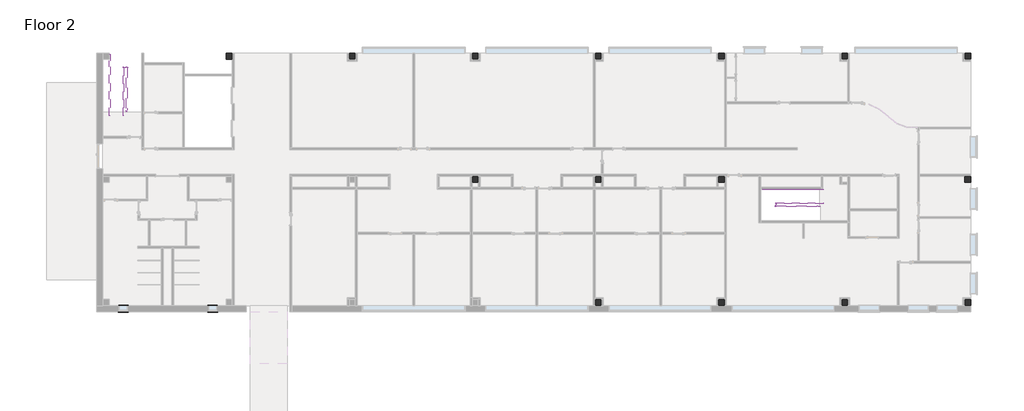
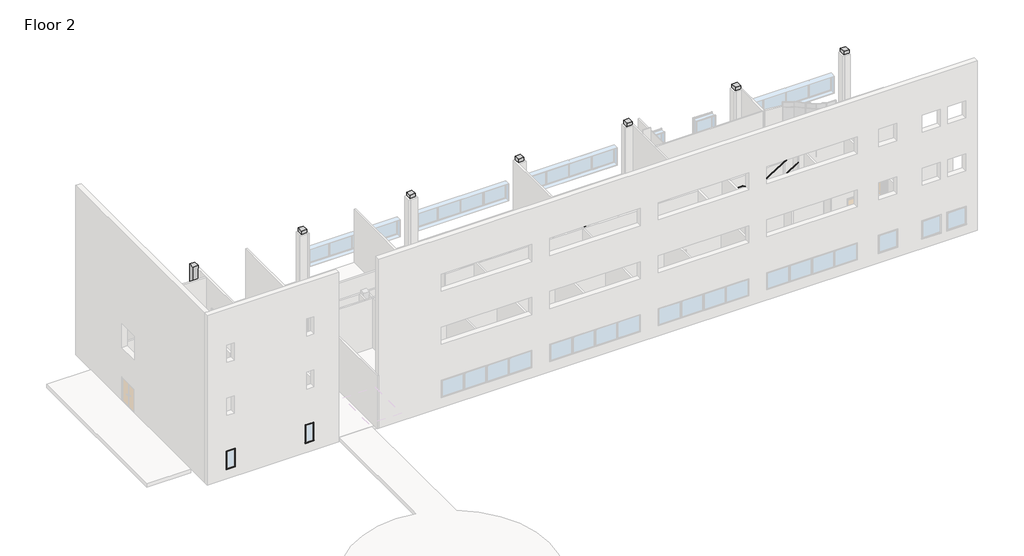
# One storey, part 5 of 7: 15 columns, 4 proxies, 4 railings.
"""IFC4 building model written with IfcOpenShell, lengths in millimetres."""

import ifcopenshell
import ifcopenshell.guid

model = None  # the IFC model being written
_history = None  # IfcOwnerHistory: only IFC2X3 demands one
_inside = {}  # id of a spatial element -> (the spatial element, [elements in it])
_under = {}  # id of a project, library or spatial element -> (it, [spatial elements below it])
_declared = {}  # id of a project -> (the project, [libraries it declares])
_typed = {}  # id of a type object -> (the type object, [elements of that type])
_made_of = {}  # id of a material, layer set ... -> (it, [elements and type objects made of it])


def new_model(schema):
    """Start an empty IFC model of exactly this schema.

    Asked for "IFC4X3", IfcOpenShell would pick the latest addendum, in which some entities
    have other attributes; the version numbers below select the first issue.
    IFC2X3 requires an IfcOwnerHistory on every rooted entity: one is made here for all.
    """
    global model, _history
    if schema == "IFC4X3":
        model = ifcopenshell.file(schema_version=(4, 3, 0, 0))
    else:
        model = ifcopenshell.file(schema=schema)
    _inside.clear()
    _under.clear()
    _declared.clear()
    _typed.clear()
    _made_of.clear()
    _history = None
    if model.schema == "IFC2X3":
        org = make("IfcOrganization", Name="unknown")
        user = make(
            "IfcPersonAndOrganization",
            ThePerson=make("IfcPerson", FamilyName="unknown"),
            TheOrganization=org,
        )
        app = make(
            "IfcApplication",
            ApplicationDeveloper=org,
            Version="unknown",
            ApplicationFullName="unknown",
            ApplicationIdentifier="unknown",
        )
        _history = make(
            "IfcOwnerHistory",
            OwningUser=user,
            OwningApplication=app,
            ChangeAction="ADDED",
            CreationDate=0,
        )
    return model


def make(cls, **values):
    """One entity of the class cls with the attributes given. An attribute that is None is left unset."""
    return model.create_entity(
        cls, **{name: value for name, value in values.items() if value is not None}
    )


def rooted(cls, **values):
    """An entity with a GlobalId (a new one), such as an element, a storey or a relation."""
    return make(cls, GlobalId=ifcopenshell.guid.new(), OwnerHistory=_history, **values)


def si_unit(unit_type, name, prefix=None):
    """IfcSIUnit, for example si_unit("LENGTHUNIT", "METRE", prefix="MILLI")."""
    return make("IfcSIUnit", UnitType=unit_type, Prefix=prefix, Name=name)


def assignment(units):
    """IfcUnitAssignment: the units of a project."""
    return None if units is None else make("IfcUnitAssignment", Units=units)


def point(xyz):
    """IfcCartesianPoint."""
    return None if xyz is None else make("IfcCartesianPoint", Coordinates=xyz)


def direction(xyz):
    """IfcDirection."""
    return None if xyz is None else make("IfcDirection", DirectionRatios=xyz)


def frame(location, z_axis=None, x_axis=None):
    """IfcAxis2Placement3D, a coordinate frame: its origin and axes. An axis left out is left unset."""
    return make(
        "IfcAxis2Placement3D",
        Location=point(location),
        Axis=direction(z_axis),
        RefDirection=direction(x_axis),
    )


def origin():
    """The frame at (0, 0, 0) with its axes left unset."""
    return frame((0.0, 0.0, 0.0))


def origin_with_axes():
    """The frame at (0, 0, 0) with the z axis (0, 0, 1) and the x axis (1, 0, 0) written out."""
    return frame((0.0, 0.0, 0.0), z_axis=(0.0, 0.0, 1.0), x_axis=(1.0, 0.0, 0.0))


def place(relative_to, where):
    """IfcLocalPlacement: puts the frame where relative to a parent placement (None: the world)."""
    return make(
        "IfcLocalPlacement", PlacementRelTo=relative_to, RelativePlacement=where
    )


def context(
    kind, dimensions, precision=None, world=None, true_north=None, identifier=None
):
    """IfcGeometricRepresentationContext, for example the 3D "Model" context."""
    return make(
        "IfcGeometricRepresentationContext",
        ContextIdentifier=identifier,
        ContextType=kind,
        CoordinateSpaceDimension=dimensions,
        Precision=precision,
        WorldCoordinateSystem=world,
        TrueNorth=true_north,
    )


def project(units=None, contexts=None):
    """IfcProject with its units and contexts."""
    return rooted(
        "IfcProject",
        Name="project",
        RepresentationContexts=contexts,
        UnitsInContext=assignment(units),
    )


def spatial(cls, under=None, at=None, **own):
    """A site, building, storey or space (cls), placed at a placement, below another one or the project."""
    s = rooted(cls, ObjectPlacement=at, **own)
    if under is not None:
        _under.setdefault(under.id(), (under, []))[1].append(s)
    return s


def polyline(points):
    """IfcPolyline through the points."""
    return make("IfcPolyline", Points=[point(p) for p in points])


def circle_curve(where, radius):
    """IfcCircle in the frame where."""
    return make("IfcCircle", Position=where, Radius=radius)


def outline(outer, holes=None, kind="AREA"):
    """IfcArbitraryClosedProfileDef: a profile drawn as a closed curve; with holes, ...WithVoids."""
    if holes is None:
        return make("IfcArbitraryClosedProfileDef", ProfileType=kind, OuterCurve=outer)
    return make(
        "IfcArbitraryProfileDefWithVoids",
        ProfileType=kind,
        OuterCurve=outer,
        InnerCurves=holes,
    )


def extrude(swept, where, along, depth):
    """IfcExtrudedAreaSolid: the profile swept, set in the frame where, extruded along a direction by depth."""
    return make(
        "IfcExtrudedAreaSolid",
        SweptArea=swept,
        Position=where,
        ExtrudedDirection=direction(along),
        Depth=depth,
    )


def faces_of(points, faces, orient=None, outer=None):
    """IfcFace entities. A face is a list of loops; a loop is a list of indices into points, from 0.

    orient and outer hold one flag for each loop. By default every Orientation is true, the
    first loop of a face is its IfcFaceOuterBound and the others are IfcFaceBound.
    """
    made = []
    for i, loops in enumerate(faces):
        bounds = []
        for j, loop in enumerate(loops):
            is_outer = j == 0 if outer is None else outer[i][j]
            bounds.append(
                make(
                    "IfcFaceOuterBound" if is_outer else "IfcFaceBound",
                    Bound=make("IfcPolyLoop", Polygon=[points[k] for k in loop]),
                    Orientation=True if orient is None else orient[i][j],
                )
            )
        made.append(make("IfcFace", Bounds=bounds))
    return made


def faceted_brep(points, faces, orient=None, outer=None, voids=None):
    """IfcFacetedBrep: a solid bounded by flat faces; with voids (closed shells), ...WithVoids."""
    shared = [point(p) for p in points]
    hull = make("IfcClosedShell", CfsFaces=faces_of(shared, faces, orient, outer))
    if voids is None:
        return make("IfcFacetedBrep", Outer=hull)
    return make(
        "IfcFacetedBrepWithVoids",
        Outer=hull,
        Voids=[
            make(cls, CfsFaces=faces_of(shared, fs, o, b)) for cls, fs, o, b in voids
        ],
    )


def shape(context_of_items, identifier, shape_type, items):
    """IfcShapeRepresentation: the items that make up one representation, for example the "Body"."""
    return make(
        "IfcShapeRepresentation",
        ContextOfItems=context_of_items,
        RepresentationIdentifier=identifier,
        RepresentationType=shape_type,
        Items=items,
    )


def source(mapping_origin, context_of_items, identifier, shape_type, items):
    """IfcRepresentationMap: a shape defined once, which mapped items show again and again."""
    return make(
        "IfcRepresentationMap",
        MappingOrigin=mapping_origin,
        MappedRepresentation=shape(context_of_items, identifier, shape_type, items),
    )


def transform(
    local_origin,
    x_axis=None,
    y_axis=None,
    z_axis=None,
    scale=None,
    scale2=None,
    scale3=None,
    uniform=True,
):
    """IfcCartesianTransformationOperator3D, or its non-uniform kind. x_axis, y_axis, z_axis: its Axis1, 2, 3."""
    if uniform:
        return make(
            "IfcCartesianTransformationOperator3D",
            Axis1=direction(x_axis),
            Axis2=direction(y_axis),
            LocalOrigin=point(local_origin),
            Scale=scale,
            Axis3=direction(z_axis),
        )
    return make(
        "IfcCartesianTransformationOperator3DnonUniform",
        Axis1=direction(x_axis),
        Axis2=direction(y_axis),
        LocalOrigin=point(local_origin),
        Scale=scale,
        Axis3=direction(z_axis),
        Scale2=scale2,
        Scale3=scale3,
    )


def mapped(mapping_source, mapping_target):
    """IfcMappedItem: shows the shape of a source again, moved by a transform."""
    return make(
        "IfcMappedItem", MappingSource=mapping_source, MappingTarget=mapping_target
    )


def made_of(thing, what):
    """Note that an element or type object is made of a material, layer set ...; save() writes the relation."""
    if what is not None:
        _made_of.setdefault(what.id(), (what, []))[1].append(thing)
    return thing


def element(
    cls,
    number,
    at=None,
    inside=None,
    cuts=None,
    type_object=None,
    material=None,
    context=None,
    identifier="Body",
    shape_type=None,
    held_by="IfcProductDefinitionShape",
    body=None,
    shapes=None,
    **own,
):
    """One element of the class cls, such as IfcWall. Its Tag is "e" and its number.

    at: its placement. inside: the storey or other place that contains it. cuts: it is an
    opening in that element (IfcRelVoidsElement). A single representation is given by context,
    identifier, shape_type and body (its items); several are given by shapes. held_by: the class
    of the entity that holds the representations. save() writes the other relations.
    """
    e = rooted(cls, Tag="e%d" % number, ObjectPlacement=at, **own)
    if body is not None:
        shapes = [shape(context, identifier, shape_type, body)]
    if shapes is not None:
        e.Representation = make(held_by, Representations=shapes)
    if inside is not None:
        _inside.setdefault(inside.id(), (inside, []))[1].append(e)
    if cuts is not None:
        rooted(
            "IfcRelVoidsElement", RelatingBuildingElement=cuts, RelatedOpeningElement=e
        )
    if type_object is not None:
        _typed.setdefault(type_object.id(), (type_object, []))[1].append(e)
    return made_of(e, material)


def aggregate(whole, parts):
    """IfcRelAggregates: a whole, such as a stair, and the parts it consists of."""
    return rooted("IfcRelAggregates", RelatingObject=whole, RelatedObjects=parts)


def save(model, path):
    """Write the relations noted so far, then the file.

    IfcRelAggregates (storeys below a building ...), IfcRelContainedInSpatialStructure (elements
    in a storey), IfcRelDefinesByType, IfcRelAssociatesMaterial and IfcRelDeclares: one each for
    every whole, place, type object, material and project.
    """
    for whole, parts in _under.values():
        aggregate(whole, parts)
    for where, things in _inside.values():
        rooted(
            "IfcRelContainedInSpatialStructure",
            RelatedElements=things,
            RelatingStructure=where,
        )
    for kind, things in _typed.values():
        rooted("IfcRelDefinesByType", RelatedObjects=things, RelatingType=kind)
    for what, things in _made_of.values():
        rooted("IfcRelAssociatesMaterial", RelatedObjects=things, RelatingMaterial=what)
    for by, libraries in _declared.values():
        rooted("IfcRelDeclares", RelatingContext=by, RelatedDefinitions=libraries)
    model.write(path)


def plane_surface(at):
    """IfcPlane: the flat surface through the origin of the frame at, square to its z axis."""
    return make("IfcPlane", Position=at)


def cylinder_surface(at, radius):
    """IfcCylindricalSurface: all points at the distance radius from the z axis of the frame at."""
    return make("IfcCylindricalSurface", Position=at, Radius=radius)


def advanced_brep(points, edges, surfaces, faces):
    """IfcAdvancedBrep: a solid bounded by faces that lie on surfaces and meet in shared edges.

    An edge is (start, end): straight between two places in points (the first is 0);
    or (start, end, curve); or (start, end, curve, False) where it runs against its curve.
    A face is (place in surfaces, loops), or (place, loops, False) where it looks against
    its surface's normal. A loop lists edges by number (the first is 1), with a minus sign
    where the edge is run from its end to its start. The first loop is the outer one.
    """
    corners = [point(p) for p in points]
    vertices = [make("IfcVertexPoint", VertexGeometry=c) for c in corners]
    made = []
    for start, end, *more in edges:
        made.append(
            make(
                "IfcEdgeCurve",
                EdgeStart=vertices[start],
                EdgeEnd=vertices[end],
                EdgeGeometry=more[0] if more else make("IfcPolyline", Points=[corners[start], corners[end]]),
                SameSense=more[1] if len(more) > 1 else True,
            )
        )
    hull = []
    for where, loops, *sense in faces:
        bounds = []
        for j, loop in enumerate(loops):
            ring = [make("IfcOrientedEdge", EdgeElement=made[abs(k) - 1], Orientation=k > 0) for k in loop]
            bounds.append(
                make(
                    "IfcFaceOuterBound" if j == 0 else "IfcFaceBound",
                    Bound=make("IfcEdgeLoop", EdgeList=ring),
                    Orientation=True,
                )
            )
        hull.append(make("IfcAdvancedFace", Bounds=bounds, FaceSurface=surfaces[where], SameSense=sense[0] if sense else True))
    return make("IfcAdvancedBrep", Outer=make("IfcClosedShell", CfsFaces=hull))


def trim_window_exterior_flat_with_sill_4912eb0d(model_context):
    return source(origin(), model_context, "Body", "SweptSolid", [
        extrude(outline(polyline([(361.95, -1546.1823709), (361.95, -1603.3323709), (-361.95, -1603.3323709), (-361.95, -1546.1823709), (361.95, -1546.1823709)])), origin_with_axes(), (0.0, 0.0, 1.0), 19.05),
        extrude(outline(polyline([(-1555.75, 38.1), (-1526.4580645, 38.1), (-1524.0, 19.05), (-1524.0, 0.0), (-1546.1823709, 0.0), (-1546.1823709, 19.05), (-1555.75, 19.05), (-1555.75, 38.1)])), frame((-374.65, 0.0, 0.0), z_axis=(1.0, 0.0, 0.0), x_axis=(0.0, 1.0, 0.0)), (0.0, 0.0, 1.0), 749.3),
        extrude(outline(polyline([(-361.95, 57.15), (361.95, 57.15), (361.95, -1524.0), (304.8, -1524.0), (304.8, 0.0), (-304.8, 0.0), (-304.8, -1524.0), (-361.95, -1524.0), (-361.95, 57.15)])), origin_with_axes(), (0.0, 0.0, 1.0), 19.05),
    ])


def trim_window_interior_flat_picture_frame_978fd00d(model_context):
    return source(origin(), model_context, "Body", "SweptSolid", [
        extrude(outline(polyline([(349.25, 44.45), (349.25, -1568.45), (-349.25, -1568.45), (-349.25, 44.45), (349.25, 44.45)]), holes=[polyline([(292.1, -12.7), (-292.1, -12.7), (-292.1, -1511.3), (292.1, -1511.3), (292.1, -12.7)])]), origin_with_axes(), (0.0, 0.0, 1.0), 31.75),
    ])


def stair_railing_1_d4a7e100(model_context):
    return source(origin(), model_context, "Body", "SolidModel", [
        faceted_brep([(-1415.3134126, 56357.2066802, 9028.2888889), (-1428.0134126, 56357.2066802, 9006.2918436), (-1453.4134126, 56357.2066802, 9006.2918436), (-1466.1134126, 56357.2066802, 9028.2888889), (-1453.4134126, 56357.2066802, 9050.2859341), (-1428.0134126, 56357.2066802, 9050.2859341), (-1415.3134126, 52725.0066802, 6753.5777778), (-1428.0134126, 52725.0066802, 6775.574823), (-1453.4134126, 52725.0066802, 6775.574823), (-1466.1134126, 52725.0066802, 6753.5777778), (-1453.4134126, 52725.0066802, 6731.5807325), (-1428.0134126, 52725.0066802, 6731.5807325)], [[[0, 1, 2, 3, 4, 5]], [[6, 7, 8, 9, 10, 11]], [[1, 0, 6, 11]], [[2, 1, 11, 10]], [[3, 2, 10, 9]], [[4, 3, 9, 8]], [[5, 4, 8, 7]], [[0, 5, 7, 6]]]),
        advanced_brep(
        [(-1136.9891104, 56281.0066802, 9028.2888889), (-1136.9891104, 56331.8066802, 9028.2888889), (-1491.5134126, 56281.0066802, 9028.2888889), (-1491.5134126, 56331.8066802, 9028.2888889)],
        [
            (0, 1, circle_curve(frame((-1136.9891104, 56306.4066802, 9028.2888889), z_axis=(1.0, 0.0, 0.0), x_axis=(0.0, -1.0, 0.0)), 25.4)),
            (1, 0, circle_curve(frame((-1136.9891104, 56306.4066802, 9028.2888889), z_axis=(1.0, 0.0, 0.0), x_axis=(0.0, -1.0, 0.0)), 25.4)),
            (2, 3, circle_curve(frame((-1491.5134126, 56306.4066802, 9028.2888889), z_axis=(-1.0, 0.0, 0.0), x_axis=(0.0, -1.0, 0.0)), 25.4)),
            (3, 2, circle_curve(frame((-1491.5134126, 56306.4066802, 9028.2888889), z_axis=(-1.0, 0.0, 0.0), x_axis=(0.0, -1.0, 0.0)), 25.4)),
            (0, 2),
            (3, 1),
        ],
        [
            plane_surface(frame((-1136.9891104, 56281.0066802, 9002.8888889), z_axis=(1.0, 0.0, 0.0), x_axis=(0.0, 1.0, 0.0))),
            plane_surface(frame((-1491.5134126, 56281.0066802, 9002.8888889), z_axis=(-1.0, 0.0, 0.0), x_axis=(0.0, -1.0, 0.0))),
            cylinder_surface(frame((-1491.5134126, 56306.4066802, 9028.2888889), z_axis=(1.0, 0.0, 0.0), x_axis=(0.0, -1.0, 0.0)), 25.4),
        ],
        [
            (0, [[1, 2]]),
            (1, [[3, 4]]),
            (2, [[-1, 5, -4, 6]]),
            (2, [[-2, -6, -3, -5]]),
        ],
    ),
        faceted_brep([(-1213.1891104, 53283.8066802, 11128.0222222), (-1200.4891104, 53283.8066802, 11106.025177), (-1175.0891104, 53283.8066802, 11106.025177), (-1162.3891104, 53283.8066802, 11128.0222222), (-1175.0891104, 53283.8066802, 11150.0192675), (-1200.4891104, 53283.8066802, 11150.0192675), (-1213.1891104, 56357.2066802, 9203.2666667), (-1200.4891104, 56357.2066802, 9225.2637119), (-1175.0891104, 56357.2066802, 9225.2637119), (-1162.3891104, 56357.2066802, 9203.2666667), (-1175.0891104, 56357.2066802, 9181.2696214), (-1200.4891104, 56357.2066802, 9181.2696214)], [[[0, 1, 2, 3, 4, 5]], [[6, 7, 8, 9, 10, 11]], [[1, 0, 6, 11]], [[2, 1, 11, 10]], [[3, 2, 10, 9]], [[4, 3, 9, 8]], [[5, 4, 8, 7]], [[0, 5, 7, 6]]]),
        faceted_brep([(-1213.1891104, 53004.4066802, 11303.0), (-1200.4891104, 53004.4066802, 11281.0029547), (-1175.0891104, 53004.4066802, 11281.0029547), (-1162.3891104, 53004.4066802, 11303.0), (-1175.0891104, 53004.4066802, 11324.9970453), (-1200.4891104, 53004.4066802, 11324.9970453), (-1213.1891104, 53283.8066802, 11128.0222222), (-1200.4891104, 53283.8066802, 11150.0192675), (-1175.0891104, 53283.8066802, 11150.0192675), (-1162.3891104, 53283.8066802, 11128.0222222), (-1175.0891104, 53283.8066802, 11106.025177), (-1200.4891104, 53283.8066802, 11106.025177)], [[[0, 1, 2, 3, 4, 5]], [[6, 7, 8, 9, 10, 11]], [[1, 0, 6, 11]], [[2, 1, 11, 10]], [[3, 2, 10, 9]], [[4, 3, 9, 8]], [[5, 4, 8, 7]], [[0, 5, 7, 6]]]),
    ])


def stair_railing_1_835fd4d1(model_context):
    return source(origin(), model_context, "Body", "SolidModel", [
        faceted_brep([(-2482.1134126, 56357.2066802, 9028.2888889), (-2469.4134126, 56357.2066802, 9050.2859341), (-2444.0134126, 56357.2066802, 9050.2859341), (-2431.3134126, 56357.2066802, 9028.2888889), (-2444.0134126, 56357.2066802, 9006.2918436), (-2469.4134126, 56357.2066802, 9006.2918436), (-2482.1134126, 52725.0066802, 6753.5777778), (-2469.4134126, 52725.0066802, 6731.5807325), (-2444.0134126, 52725.0066802, 6731.5807325), (-2431.3134126, 52725.0066802, 6753.5777778), (-2444.0134126, 52725.0066802, 6775.574823), (-2469.4134126, 52725.0066802, 6775.574823)], [[[0, 1, 2, 3, 4, 5]], [[6, 7, 8, 9, 10, 11]], [[1, 0, 6, 11]], [[2, 1, 11, 10]], [[3, 2, 10, 9]], [[4, 3, 9, 8]], [[5, 4, 8, 7]], [[0, 5, 7, 6]]]),
        advanced_brep(
        [(-2482.1134126, 57271.6066802, 9028.2888889), (-2431.3134126, 57271.6066802, 9028.2888889), (-2482.1134126, 56357.2066802, 9028.2888889), (-2431.3134126, 56357.2066802, 9028.2888889)],
        [
            (0, 1, circle_curve(frame((-2456.7134126, 57271.6066802, 9028.2888889), z_axis=(0.0, 1.0, 0.0), x_axis=(-0.9999999999999999, 0.0, 0.0)), 25.4)),
            (1, 0, circle_curve(frame((-2456.7134126, 57271.6066802, 9028.2888889), z_axis=(0.0, 1.0, 0.0), x_axis=(-0.9999999999999999, 0.0, 0.0)), 25.4)),
            (2, 3, circle_curve(frame((-2456.7134126, 56357.2066802, 9028.2888889), z_axis=(0.0, -1.0, 0.0), x_axis=(-0.9999999999999999, 0.0, 0.0)), 25.4)),
            (3, 2, circle_curve(frame((-2456.7134126, 56357.2066802, 9028.2888889), z_axis=(0.0, -1.0, 0.0), x_axis=(-0.9999999999999999, 0.0, 0.0)), 25.4)),
            (0, 2),
            (3, 1),
        ],
        [
            plane_surface(frame((-2482.1134126, 57271.6066802, 9002.8888889), z_axis=(0.0, 1.0, 0.0), x_axis=(0.0, 0.0, 1.0))),
            plane_surface(frame((-2482.1134126, 56357.2066802, 9002.8888889), z_axis=(0.0, -1.0, 0.0), x_axis=(0.0, 0.0, -1.0))),
            cylinder_surface(frame((-2456.7134126, 56357.2066802, 9028.2888889), z_axis=(0.0, 0.9999999999999999, 0.0), x_axis=(-0.9999999999999999, 0.0, 0.0)), 25.4),
        ],
        [
            (0, [[1, 2]]),
            (1, [[3, 4]]),
            (2, [[-1, 5, -4, 6]]),
            (2, [[-2, -6, -3, -5]]),
        ],
    ),
        advanced_brep(
        [(-222.5891104, 57347.8066802, 9028.2888889), (-222.5891104, 57297.0066802, 9028.2888889), (-2405.9134126, 57347.8066802, 9028.2888889), (-2405.9134126, 57297.0066802, 9028.2888889)],
        [
            (0, 1, circle_curve(frame((-222.5891104, 57322.4066802, 9028.2888889), z_axis=(1.0, 0.0, 0.0), x_axis=(0.0, 1.0, 0.0)), 25.4)),
            (1, 0, circle_curve(frame((-222.5891104, 57322.4066802, 9028.2888889), z_axis=(1.0, 0.0, 0.0), x_axis=(0.0, 1.0, 0.0)), 25.4)),
            (2, 3, circle_curve(frame((-2405.9134126, 57322.4066802, 9028.2888889), z_axis=(-1.0, 0.0, 0.0), x_axis=(0.0, 1.0, 0.0)), 25.4)),
            (3, 2, circle_curve(frame((-2405.9134126, 57322.4066802, 9028.2888889), z_axis=(-1.0, 0.0, 0.0), x_axis=(0.0, 1.0, 0.0)), 25.4)),
            (0, 2),
            (3, 1),
        ],
        [
            plane_surface(frame((-222.5891104, 57347.8066802, 9002.8888889), z_axis=(1.0, 0.0, 0.0), x_axis=(0.0, 1.0, 0.0))),
            plane_surface(frame((-2405.9134126, 57347.8066802, 9002.8888889), z_axis=(-1.0, 0.0, 0.0), x_axis=(0.0, -1.0, 0.0))),
            cylinder_surface(frame((-2405.9134126, 57322.4066802, 9028.2888889), z_axis=(1.0, 0.0, 0.0), x_axis=(0.0, 1.0, 0.0)), 25.4),
        ],
        [
            (0, [[1, 2]]),
            (1, [[3, 4]]),
            (2, [[-1, 5, -4, 6]]),
            (2, [[-2, -6, -3, -5]]),
        ],
    ),
        advanced_brep(
        [(-146.3891104, 56636.6066802, 9028.2888889), (-197.1891104, 56636.6066802, 9028.2888889), (-146.3891104, 57271.6066802, 9028.2888889), (-197.1891104, 57271.6066802, 9028.2888889)],
        [
            (0, 1, circle_curve(frame((-171.7891104, 56636.6066802, 9028.2888889), z_axis=(0.0, -1.0, 0.0), x_axis=(1.0, 0.0, 0.0)), 25.4)),
            (1, 0, circle_curve(frame((-171.7891104, 56636.6066802, 9028.2888889), z_axis=(0.0, -1.0, 0.0), x_axis=(1.0, 0.0, 0.0)), 25.4)),
            (2, 3, circle_curve(frame((-171.7891104, 57271.6066802, 9028.2888889), z_axis=(0.0, 1.0, 0.0), x_axis=(1.0, 0.0, 0.0)), 25.4)),
            (3, 2, circle_curve(frame((-171.7891104, 57271.6066802, 9028.2888889), z_axis=(0.0, 1.0, 0.0), x_axis=(1.0, 0.0, 0.0)), 25.4)),
            (0, 2),
            (3, 1),
        ],
        [
            plane_surface(frame((-146.3891104, 56636.6066802, 9002.8888889), z_axis=(0.0, -1.0, 0.0), x_axis=(0.0, 0.0, -1.0))),
            plane_surface(frame((-146.3891104, 57271.6066802, 9002.8888889), z_axis=(0.0, 1.0, 0.0), x_axis=(0.0, 0.0, 1.0))),
            cylinder_surface(frame((-171.7891104, 57271.6066802, 9028.2888889), z_axis=(0.0, -1.0, 0.0), x_axis=(1.0, 0.0, 0.0)), 25.4),
        ],
        [
            (0, [[1, 2]]),
            (1, [[3, 4]]),
            (2, [[-1, 5, -4, 6]]),
            (2, [[-2, -6, -3, -5]]),
        ],
    ),
        faceted_brep([(-146.3891104, 56357.2066802, 9203.2666667), (-159.0891104, 56357.2066802, 9225.2637119), (-184.4891104, 56357.2066802, 9225.2637119), (-197.1891104, 56357.2066802, 9203.2666667), (-184.4891104, 56357.2066802, 9181.2696214), (-159.0891104, 56357.2066802, 9181.2696214), (-146.3891104, 56636.6066802, 9028.2888889), (-159.0891104, 56636.6066802, 9006.2918436), (-184.4891104, 56636.6066802, 9006.2918436), (-197.1891104, 56636.6066802, 9028.2888889), (-184.4891104, 56636.6066802, 9050.2859341), (-159.0891104, 56636.6066802, 9050.2859341)], [[[0, 1, 2, 3, 4, 5]], [[6, 7, 8, 9, 10, 11]], [[1, 0, 6, 11]], [[2, 1, 11, 10]], [[3, 2, 10, 9]], [[4, 3, 9, 8]], [[5, 4, 8, 7]], [[0, 5, 7, 6]]]),
        faceted_brep([(-146.3891104, 53283.8066802, 11128.0222222), (-159.0891104, 53283.8066802, 11150.0192675), (-184.4891104, 53283.8066802, 11150.0192675), (-197.1891104, 53283.8066802, 11128.0222222), (-184.4891104, 53283.8066802, 11106.025177), (-159.0891104, 53283.8066802, 11106.025177), (-146.3891104, 56357.2066802, 9203.2666667), (-159.0891104, 56357.2066802, 9181.2696214), (-184.4891104, 56357.2066802, 9181.2696214), (-197.1891104, 56357.2066802, 9203.2666667), (-184.4891104, 56357.2066802, 9225.2637119), (-159.0891104, 56357.2066802, 9225.2637119)], [[[0, 1, 2, 3, 4, 5]], [[6, 7, 8, 9, 10, 11]], [[1, 0, 6, 11]], [[2, 1, 11, 10]], [[3, 2, 10, 9]], [[4, 3, 9, 8]], [[5, 4, 8, 7]], [[0, 5, 7, 6]]]),
        faceted_brep([(-146.3891104, 53004.4066802, 11303.0), (-159.0891104, 53004.4066802, 11324.9970453), (-184.4891104, 53004.4066802, 11324.9970453), (-197.1891104, 53004.4066802, 11303.0), (-184.4891104, 53004.4066802, 11281.0029547), (-159.0891104, 53004.4066802, 11281.0029547), (-146.3891104, 53283.8066802, 11128.0222222), (-159.0891104, 53283.8066802, 11106.025177), (-184.4891104, 53283.8066802, 11106.025177), (-197.1891104, 53283.8066802, 11128.0222222), (-184.4891104, 53283.8066802, 11150.0192675), (-159.0891104, 53283.8066802, 11150.0192675)], [[[0, 1, 2, 3, 4, 5]], [[6, 7, 8, 9, 10, 11]], [[1, 0, 6, 11]], [[2, 1, 11, 10]], [[3, 2, 10, 9]], [[4, 3, 9, 8]], [[5, 4, 8, 7]], [[0, 5, 7, 6]]]),
    ])


def stair_railing_1_a30edcdb(model_context):
    return source(origin(), model_context, "Body", "SolidModel", [
        faceted_brep([(46974.7398084, 47258.2865351, 9028.2888889), (46974.7398084, 47245.5865351, 9006.2918436), (46974.7398084, 47220.1865351, 9006.2918436), (46974.7398084, 47207.4865351, 9028.2888889), (46974.7398084, 47220.1865351, 9050.2859341), (46974.7398084, 47245.5865351, 9050.2859341), (50533.2139908, 47258.2865351, 6753.5777778), (50533.2139908, 47245.5865351, 6775.574823), (50533.2139908, 47220.1865351, 6775.574823), (50533.2139908, 47207.4865351, 6753.5777778), (50533.2139908, 47220.1865351, 6731.5807325), (50533.2139908, 47245.5865351, 6731.5807325)], [[[0, 1, 2, 3, 4, 5]], [[6, 7, 8, 9, 10, 11]], [[1, 0, 6, 11]], [[2, 1, 11, 10]], [[3, 2, 10, 9]], [[4, 3, 9, 8]], [[5, 4, 8, 7]], [[0, 5, 7, 6]]]),
        advanced_brep(
        [(46060.3398084, 47258.2865351, 9028.2888889), (46060.3398084, 47207.4865351, 9028.2888889), (46974.7398084, 47258.2865351, 9028.2888889), (46974.7398084, 47207.4865351, 9028.2888889)],
        [
            (0, 1, circle_curve(frame((46060.3398084, 47232.8865351, 9028.2888889), z_axis=(-1.0, 0.0, 0.0), x_axis=(0.0, 1.0, 0.0)), 25.4)),
            (1, 0, circle_curve(frame((46060.3398084, 47232.8865351, 9028.2888889), z_axis=(-1.0, 0.0, 0.0), x_axis=(0.0, 1.0, 0.0)), 25.4)),
            (2, 3, circle_curve(frame((46974.7398084, 47232.8865351, 9028.2888889), z_axis=(1.0, 0.0, 0.0), x_axis=(0.0, 1.0, 0.0)), 25.4)),
            (3, 2, circle_curve(frame((46974.7398084, 47232.8865351, 9028.2888889), z_axis=(1.0, 0.0, 0.0), x_axis=(0.0, 1.0, 0.0)), 25.4)),
            (0, 2),
            (3, 1),
        ],
        [
            plane_surface(frame((46060.3398084, 47258.2865351, 9002.8888889), z_axis=(-1.0, 0.0, 0.0), x_axis=(0.0, -1.0, 0.0))),
            plane_surface(frame((46974.7398084, 47258.2865351, 9002.8888889), z_axis=(1.0, 0.0, 0.0), x_axis=(0.0, 1.0, 0.0))),
            cylinder_surface(frame((46974.7398084, 47232.8865351, 9028.2888889), z_axis=(-1.0, 0.0, 0.0), x_axis=(0.0, 1.0, 0.0)), 25.4),
        ],
        [
            (0, [[1, 2]]),
            (1, [[3, 4]]),
            (2, [[-1, 5, -4, 6]]),
            (2, [[-2, -6, -3, -5]]),
        ],
    ),
        advanced_brep(
        [(45984.1398084, 45032.0030566, 9028.2888889), (46034.9398084, 45032.0030566, 9028.2888889), (45984.1398084, 47182.0865351, 9028.2888889), (46034.9398084, 47182.0865351, 9028.2888889)],
        [
            (0, 1, circle_curve(frame((46009.5398084, 45032.0030566, 9028.2888889), z_axis=(0.0, -1.0, 0.0), x_axis=(-1.0, 0.0, 0.0)), 25.4)),
            (1, 0, circle_curve(frame((46009.5398084, 45032.0030566, 9028.2888889), z_axis=(0.0, -1.0, 0.0), x_axis=(-1.0, 0.0, 0.0)), 25.4)),
            (2, 3, circle_curve(frame((46009.5398084, 47182.0865351, 9028.2888889), z_axis=(0.0, 1.0, 0.0), x_axis=(-1.0, 0.0, 0.0)), 25.4)),
            (3, 2, circle_curve(frame((46009.5398084, 47182.0865351, 9028.2888889), z_axis=(0.0, 1.0, 0.0), x_axis=(-1.0, 0.0, 0.0)), 25.4)),
            (0, 2),
            (3, 1),
        ],
        [
            plane_surface(frame((45984.1398084, 45032.0030566, 9002.8888889), z_axis=(0.0, -1.0, 0.0), x_axis=(0.0, 0.0, -1.0))),
            plane_surface(frame((45984.1398084, 47182.0865351, 9002.8888889), z_axis=(0.0, 1.0, 0.0), x_axis=(0.0, 0.0, 1.0))),
            cylinder_surface(frame((46009.5398084, 47182.0865351, 9028.2888889), z_axis=(0.0, -1.0, 0.0), x_axis=(-1.0, 0.0, 0.0)), 25.4),
        ],
        [
            (0, [[1, 2]]),
            (1, [[3, 4]]),
            (2, [[-1, 5, -4, 6]]),
            (2, [[-2, -6, -3, -5]]),
        ],
    ),
        advanced_brep(
        [(46695.3398084, 44955.8030566, 9028.2888889), (46695.3398084, 45006.6030566, 9028.2888889), (46060.3398084, 44955.8030566, 9028.2888889), (46060.3398084, 45006.6030566, 9028.2888889)],
        [
            (0, 1, circle_curve(frame((46695.3398084, 44981.2030566, 9028.2888889), z_axis=(1.0, 0.0, 0.0), x_axis=(0.0, -1.0, 0.0)), 25.4)),
            (1, 0, circle_curve(frame((46695.3398084, 44981.2030566, 9028.2888889), z_axis=(1.0, 0.0, 0.0), x_axis=(0.0, -1.0, 0.0)), 25.4)),
            (2, 3, circle_curve(frame((46060.3398084, 44981.2030566, 9028.2888889), z_axis=(-1.0, 0.0, 0.0), x_axis=(0.0, -1.0, 0.0)), 25.4)),
            (3, 2, circle_curve(frame((46060.3398084, 44981.2030566, 9028.2888889), z_axis=(-1.0, 0.0, 0.0), x_axis=(0.0, -1.0, 0.0)), 25.4)),
            (0, 2),
            (3, 1),
        ],
        [
            plane_surface(frame((46695.3398084, 44955.8030566, 9002.8888889), z_axis=(1.0, 0.0, 0.0), x_axis=(0.0, 1.0, 0.0))),
            plane_surface(frame((46060.3398084, 44955.8030566, 9002.8888889), z_axis=(-1.0, 0.0, 0.0), x_axis=(0.0, -1.0, 0.0))),
            cylinder_surface(frame((46060.3398084, 44981.2030566, 9028.2888889), z_axis=(1.0, 0.0, 0.0), x_axis=(0.0, -1.0, 0.0)), 25.4),
        ],
        [
            (0, [[1, 2]]),
            (1, [[3, 4]]),
            (2, [[-1, 5, -4, 6]]),
            (2, [[-2, -6, -3, -5]]),
        ],
    ),
        faceted_brep([(46974.7398084, 44955.8030566, 9203.2666667), (46974.7398084, 44968.5030566, 9181.2696214), (46974.7398084, 44993.9030566, 9181.2696214), (46974.7398084, 45006.6030566, 9203.2666667), (46974.7398084, 44993.9030566, 9225.2637119), (46974.7398084, 44968.5030566, 9225.2637119), (46695.3398084, 44955.8030566, 9028.2888889), (46695.3398084, 44968.5030566, 9050.2859341), (46695.3398084, 44993.9030566, 9050.2859341), (46695.3398084, 45006.6030566, 9028.2888889), (46695.3398084, 44993.9030566, 9006.2918436), (46695.3398084, 44968.5030566, 9006.2918436)], [[[0, 1, 2, 3, 4, 5]], [[6, 7, 8, 9, 10, 11]], [[1, 0, 6, 11]], [[2, 1, 11, 10]], [[3, 2, 10, 9]], [[4, 3, 9, 8]], [[5, 4, 8, 7]], [[0, 5, 7, 6]]]),
        faceted_brep([(50048.1398084, 44955.8030566, 11128.0222222), (50048.1398084, 44968.5030566, 11106.025177), (50048.1398084, 44993.9030566, 11106.025177), (50048.1398084, 45006.6030566, 11128.0222222), (50048.1398084, 44993.9030566, 11150.0192675), (50048.1398084, 44968.5030566, 11150.0192675), (46974.7398084, 44955.8030566, 9203.2666667), (46974.7398084, 44968.5030566, 9225.2637119), (46974.7398084, 44993.9030566, 9225.2637119), (46974.7398084, 45006.6030566, 9203.2666667), (46974.7398084, 44993.9030566, 9181.2696214), (46974.7398084, 44968.5030566, 9181.2696214)], [[[0, 1, 2, 3, 4, 5]], [[6, 7, 8, 9, 10, 11]], [[1, 0, 6, 11]], [[2, 1, 11, 10]], [[3, 2, 10, 9]], [[4, 3, 9, 8]], [[5, 4, 8, 7]], [[0, 5, 7, 6]]]),
        faceted_brep([(50327.5398084, 44955.8030566, 11303.0), (50327.5398084, 44968.5030566, 11281.0029547), (50327.5398084, 44993.9030566, 11281.0029547), (50327.5398084, 45006.6030566, 11303.0), (50327.5398084, 44993.9030566, 11324.9970453), (50327.5398084, 44968.5030566, 11324.9970453), (50048.1398084, 44955.8030566, 11128.0222222), (50048.1398084, 44968.5030566, 11150.0192675), (50048.1398084, 44993.9030566, 11150.0192675), (50048.1398084, 45006.6030566, 11128.0222222), (50048.1398084, 44993.9030566, 11106.025177), (50048.1398084, 44968.5030566, 11106.025177)], [[[0, 1, 2, 3, 4, 5]], [[6, 7, 8, 9, 10, 11]], [[1, 0, 6, 11]], [[2, 1, 11, 10]], [[3, 2, 10, 9]], [[4, 3, 9, 8]], [[5, 4, 8, 7]], [[0, 5, 7, 6]]]),
    ])


def stair_railing_1_ea28da98(model_context):
    return source(origin(), model_context, "Body", "SolidModel", [
        faceted_brep([(46974.7398084, 46191.4865351, 9028.2888889), (46974.7398084, 46204.1865351, 9050.2859341), (46974.7398084, 46229.5865351, 9050.2859341), (46974.7398084, 46242.2865351, 9028.2888889), (46974.7398084, 46229.5865351, 9006.2918436), (46974.7398084, 46204.1865351, 9006.2918436), (50533.2139908, 46191.4865351, 6753.5777778), (50533.2139908, 46204.1865351, 6731.5807325), (50533.2139908, 46229.5865351, 6731.5807325), (50533.2139908, 46242.2865351, 6753.5777778), (50533.2139908, 46229.5865351, 6775.574823), (50533.2139908, 46204.1865351, 6775.574823)], [[[0, 1, 2, 3, 4, 5]], [[6, 7, 8, 9, 10, 11]], [[1, 0, 6, 11]], [[2, 1, 11, 10]], [[3, 2, 10, 9]], [[4, 3, 9, 8]], [[5, 4, 8, 7]], [[0, 5, 7, 6]]]),
        advanced_brep(
        [(47050.9398084, 45946.4030566, 9028.2888889), (47000.1398084, 45946.4030566, 9028.2888889), (47050.9398084, 46267.6865351, 9028.2888889), (47000.1398084, 46267.6865351, 9028.2888889)],
        [
            (0, 1, circle_curve(frame((47025.5398084, 45946.4030566, 9028.2888889), z_axis=(0.0, -1.0, 0.0), x_axis=(1.0, 0.0, 0.0)), 25.4)),
            (1, 0, circle_curve(frame((47025.5398084, 45946.4030566, 9028.2888889), z_axis=(0.0, -1.0, 0.0), x_axis=(1.0, 0.0, 0.0)), 25.4)),
            (2, 3, circle_curve(frame((47025.5398084, 46267.6865351, 9028.2888889), z_axis=(0.0, 1.0, 0.0), x_axis=(1.0, 0.0, 0.0)), 25.4)),
            (3, 2, circle_curve(frame((47025.5398084, 46267.6865351, 9028.2888889), z_axis=(0.0, 1.0, 0.0), x_axis=(1.0, 0.0, 0.0)), 25.4)),
            (0, 2),
            (3, 1),
        ],
        [
            plane_surface(frame((47050.9398084, 45946.4030566, 9002.8888889), z_axis=(0.0, -1.0, 0.0), x_axis=(0.0, 0.0, -1.0))),
            plane_surface(frame((47050.9398084, 46267.6865351, 9002.8888889), z_axis=(0.0, 1.0, 0.0), x_axis=(0.0, 0.0, 1.0))),
            cylinder_surface(frame((47025.5398084, 46267.6865351, 9028.2888889), z_axis=(0.0, -1.0, 0.0), x_axis=(1.0, 0.0, 0.0)), 25.4),
        ],
        [
            (0, [[1, 2]]),
            (1, [[3, 4]]),
            (2, [[-1, 5, -4, 6]]),
            (2, [[-2, -6, -3, -5]]),
        ],
    ),
        faceted_brep([(50048.1398084, 46022.6030566, 11128.0222222), (50048.1398084, 46009.9030566, 11150.0192675), (50048.1398084, 45984.5030566, 11150.0192675), (50048.1398084, 45971.8030566, 11128.0222222), (50048.1398084, 45984.5030566, 11106.025177), (50048.1398084, 46009.9030566, 11106.025177), (46974.7398084, 46022.6030566, 9203.2666667), (46974.7398084, 46009.9030566, 9181.2696214), (46974.7398084, 45984.5030566, 9181.2696214), (46974.7398084, 45971.8030566, 9203.2666667), (46974.7398084, 45984.5030566, 9225.2637119), (46974.7398084, 46009.9030566, 9225.2637119)], [[[0, 1, 2, 3, 4, 5]], [[6, 7, 8, 9, 10, 11]], [[1, 0, 6, 11]], [[2, 1, 11, 10]], [[3, 2, 10, 9]], [[4, 3, 9, 8]], [[5, 4, 8, 7]], [[0, 5, 7, 6]]]),
        faceted_brep([(50327.5398084, 46022.6030566, 11303.0), (50327.5398084, 46009.9030566, 11324.9970453), (50327.5398084, 45984.5030566, 11324.9970453), (50327.5398084, 45971.8030566, 11303.0), (50327.5398084, 45984.5030566, 11281.0029547), (50327.5398084, 46009.9030566, 11281.0029547), (50048.1398084, 46022.6030566, 11128.0222222), (50048.1398084, 46009.9030566, 11106.025177), (50048.1398084, 45984.5030566, 11106.025177), (50048.1398084, 45971.8030566, 11128.0222222), (50048.1398084, 45984.5030566, 11150.0192675), (50048.1398084, 46009.9030566, 11150.0192675)], [[[0, 1, 2, 3, 4, 5]], [[6, 7, 8, 9, 10, 11]], [[1, 0, 6, 11]], [[2, 1, 11, 10]], [[3, 2, 10, 9]], [[4, 3, 9, 8]], [[5, 4, 8, 7]], [[0, 5, 7, 6]]]),
    ])


model = new_model("IFC4")

# Units and contexts
model_context = context("Model", 3, world=origin())
ifc_project = project(units=[si_unit("LENGTHUNIT", "METRE", prefix="MILLI")], contexts=[model_context])

# Site, building, storey
site = spatial("IfcSite", under=ifc_project)
building = spatial("IfcBuilding", under=site)
storey = spatial("IfcBuildingStorey", under=building, Name="Floor 2", Elevation=5486.4)

# Proxies
placement = place(None, origin())
trim_window_exterior_flat_with_sill_shape = trim_window_exterior_flat_with_sill_4912eb0d(model_context)
element("IfcBuildingElementProxy", 1, Name="Trim-Window-Exterior-Flat : with Sill", ObjectType="Trim-Window-Exterior-Flat : with Sill", at=placement, inside=storey, context=model_context, shape_type="MappedRepresentation", body=[
    mapped(trim_window_exterior_flat_with_sill_shape, transform((-1446.1807976, 38164.299389, 7924.8), x_axis=(1.0, 0.0, 0.0), y_axis=(0.0, 0.0, 1.0), z_axis=(0.0, -1.0, 0.0))),
])
element("IfcBuildingElementProxy", 2, Name="Trim-Window-Exterior-Flat : with Sill", ObjectType="Trim-Window-Exterior-Flat : with Sill", at=placement, inside=storey, context=model_context, shape_type="MappedRepresentation", body=[
    mapped(trim_window_exterior_flat_with_sill_shape, transform((5189.5692024, 38164.299389, 7924.8), x_axis=(1.0, 0.0, 0.0), y_axis=(0.0, 0.0, 1.0), z_axis=(0.0, -1.0, 0.0))),
])
trim_window_interior_flat_picture_frame_shape = trim_window_interior_flat_picture_frame_978fd00d(model_context)
element("IfcBuildingElementProxy", 3, Name="Trim-Window-Interior-Flat : Picture Frame", ObjectType="Trim-Window-Interior-Flat : Picture Frame", at=placement, inside=storey, context=model_context, shape_type="MappedRepresentation", body=[
    mapped(trim_window_interior_flat_picture_frame_shape, transform((-1446.1807976, 38618.324389, 7924.8), x_axis=(-1.0, 0.0, 0.0), y_axis=(0.0, 0.0, 1.0), z_axis=(0.0, 1.0, 0.0))),
])
element("IfcBuildingElementProxy", 4, Name="Trim-Window-Interior-Flat : Picture Frame", ObjectType="Trim-Window-Interior-Flat : Picture Frame", at=placement, inside=storey, context=model_context, shape_type="MappedRepresentation", body=[
    mapped(trim_window_interior_flat_picture_frame_shape, transform((5189.5692024, 38618.324389, 7924.8), x_axis=(-1.0, 0.0, 0.0), y_axis=(0.0, 0.0, 1.0), z_axis=(0.0, 1.0, 0.0))),
])

# Columns
element("IfcColumn", 5, ObjectType="Rectangular Column1 : 18\" x 18\"", at=placement, inside=storey, context=model_context, shape_type="Brep", body=[
    faceted_brep([(34069.3692024, 39077.111889, 10210.8), (33612.1692024, 39077.111889, 10210.8), (33612.1692024, 38619.911889, 10210.8), (34069.3692024, 38619.911889, 10210.8), (34069.3692024, 39077.111889, 5486.4), (34069.3692024, 38619.911889, 5486.4), (33612.1692024, 38619.911889, 5486.4), (33612.1692024, 39077.111889, 5486.4), (34069.3692024, 39077.111889, 9906.0), (33612.1692024, 39077.111889, 9906.0)], [[[0, 1, 2, 3]], [[4, 5, 6, 7]], [[1, 0, 8, 4, 7, 9]], [[2, 1, 9, 7, 6]], [[3, 2, 6, 5]], [[0, 3, 5, 4, 8]]]),
])
element("IfcColumn", 6, ObjectType="Rectangular Column1 : 18\" x 18\"", at=placement, inside=storey, context=model_context, shape_type="Brep", body=[
    faceted_brep([(43213.3692024, 39077.111889, 10210.8), (42756.1692024, 39077.111889, 10210.8), (42756.1692024, 38619.911889, 10210.8), (43213.3692024, 38619.911889, 10210.8), (43213.3692024, 39077.111889, 5486.4), (43213.3692024, 38619.911889, 5486.4), (42756.1692024, 38619.911889, 5486.4), (42756.1692024, 39077.111889, 5486.4), (43213.3692024, 39077.111889, 9906.0), (42756.1692024, 39077.111889, 9906.0)], [[[0, 1, 2, 3]], [[4, 5, 6, 7]], [[1, 0, 8, 4, 7, 9]], [[2, 1, 9, 7, 6]], [[3, 2, 6, 5]], [[0, 3, 5, 4, 8]]]),
])
element("IfcColumn", 7, ObjectType="Rectangular Column1 : 18\" x 18\"", at=placement, inside=storey, context=model_context, shape_type="Brep", body=[
    faceted_brep([(52357.3692024, 39077.111889, 10210.8), (51900.1692024, 39077.111889, 10210.8), (51900.1692024, 38619.911889, 10210.8), (52357.3692024, 38619.911889, 10210.8), (52357.3692024, 39077.111889, 5486.4), (52357.3692024, 38619.911889, 5486.4), (51900.1692024, 38619.911889, 5486.4), (51900.1692024, 39077.111889, 5486.4), (52357.3692024, 39077.111889, 9906.0), (51900.1692024, 39077.111889, 9906.0)], [[[0, 1, 2, 3]], [[4, 5, 6, 7]], [[1, 0, 8, 4, 7, 9]], [[2, 1, 9, 7, 6]], [[3, 2, 6, 5]], [[0, 3, 5, 4, 8]]]),
])
element("IfcColumn", 8, ObjectType="Rectangular Column1 : 18\" x 18\"", at=placement, inside=storey, context=model_context, shape_type="Brep", body=[
    faceted_brep([(61501.3692024, 39077.111889, 10210.8), (61044.1692024, 39077.111889, 10210.8), (61044.1692024, 38619.911889, 10210.8), (61501.3692024, 38619.911889, 10210.8), (61501.3692024, 39077.111889, 5486.4), (61501.3692024, 38619.911889, 5486.4), (61044.1692024, 38619.911889, 5486.4), (61044.1692024, 39077.111889, 5486.4), (61044.1692024, 39077.111889, 9906.0)], [[[0, 1, 2, 3]], [[4, 5, 6, 7]], [[1, 0, 4, 7, 8]], [[2, 1, 8, 7, 6]], [[3, 2, 6, 5]], [[0, 3, 5, 4]]]),
])
element("IfcColumn", 9, ObjectType="Rectangular Column1 : 18\" x 18\"", at=placement, inside=storey, context=model_context, shape_type="Brep", body=[
    faceted_brep([(24925.3692024, 48221.111889, 10210.8), (24468.1692024, 48221.111889, 10210.8), (24468.1692024, 47763.911889, 10210.8), (24925.3692024, 47763.911889, 10210.8), (24925.3692024, 48221.111889, 5486.4), (24925.3692024, 47763.911889, 5486.4), (24468.1692024, 47763.911889, 5486.4), (24468.1692024, 48221.111889, 5486.4), (24925.3692024, 48221.111889, 9906.0), (24468.1692024, 48221.111889, 9906.0)], [[[0, 1, 2, 3]], [[4, 5, 6, 7]], [[1, 0, 8, 4, 7, 9]], [[2, 1, 9, 7, 6]], [[3, 2, 6, 5]], [[0, 3, 5, 4, 8]]]),
])
element("IfcColumn", 10, ObjectType="Rectangular Column1 : 18\" x 18\"", at=placement, inside=storey, context=model_context, shape_type="Brep", body=[
    faceted_brep([(34069.3692024, 48221.111889, 10210.8), (33612.1692024, 48221.111889, 10210.8), (33612.1692024, 47763.911889, 10210.8), (34069.3692024, 47763.911889, 10210.8), (34069.3692024, 48221.111889, 5486.4), (34069.3692024, 47763.911889, 5486.4), (33612.1692024, 47763.911889, 5486.4), (33612.1692024, 48221.111889, 5486.4), (34069.3692024, 48221.111889, 9906.0), (33612.1692024, 48221.111889, 9906.0)], [[[0, 1, 2, 3]], [[4, 5, 6, 7]], [[1, 0, 8, 4, 7, 9]], [[2, 1, 9, 7, 6]], [[3, 2, 6, 5]], [[0, 3, 5, 4, 8]]]),
])
element("IfcColumn", 11, ObjectType="Rectangular Column1 : 18\" x 18\"", at=placement, inside=storey, context=model_context, shape_type="Brep", body=[
    faceted_brep([(43213.3692024, 48221.111889, 10210.8), (42756.1692024, 48221.111889, 10210.8), (42756.1692024, 47763.911889, 10210.8), (43213.3692024, 47763.911889, 10210.8), (43213.3692024, 48221.111889, 5486.4), (43213.3692024, 47763.911889, 5486.4), (42756.1692024, 47763.911889, 5486.4), (42756.1692024, 48221.111889, 5486.4), (43213.3692024, 48221.111889, 9906.0), (42756.1692024, 48221.111889, 9906.0)], [[[0, 1, 2, 3]], [[4, 5, 6, 7]], [[1, 0, 8, 4, 7, 9]], [[2, 1, 9, 7, 6]], [[3, 2, 6, 5]], [[0, 3, 5, 4, 8]]]),
])
element("IfcColumn", 12, ObjectType="Rectangular Column1 : 18\" x 18\"", at=placement, inside=storey, context=model_context, shape_type="SweptSolid", body=[
    extrude(outline(polyline([(61501.3692024, 48221.111889), (61501.3692024, 47763.911889), (61044.1692024, 47763.911889), (61044.1692024, 48221.111889), (61501.3692024, 48221.111889)])), frame((0.0, 0.0, 5486.4), z_axis=(0.0, 0.0, 1.0), x_axis=(1.0, 0.0, 0.0)), (0.0, 0.0, 1.0), 4724.4),
])
element("IfcColumn", 13, ObjectType="Rectangular Column1 : 18\" x 18\"", at=placement, inside=storey, context=model_context, shape_type="SweptSolid", body=[
    extrude(outline(polyline([(6637.3692024, 57365.111889), (6637.3692024, 56907.911889), (6180.1692024, 56907.911889), (6180.1692024, 57365.111889), (6637.3692024, 57365.111889)])), frame((0.0, 0.0, 5486.4), z_axis=(0.0, 0.0, 1.0), x_axis=(1.0, 0.0, 0.0)), (0.0, 0.0, 1.0), 4724.4),
])
element("IfcColumn", 14, ObjectType="Rectangular Column1 : 18\" x 18\"", at=placement, inside=storey, context=model_context, shape_type="Brep", body=[
    faceted_brep([(15781.3692024, 57365.111889, 10210.8), (15324.1692024, 57365.111889, 10210.8), (15324.1692024, 56907.911889, 10210.8), (15781.3692024, 56907.911889, 10210.8), (15781.3692024, 57365.111889, 5486.4), (15781.3692024, 56907.911889, 5486.4), (15324.1692024, 56907.911889, 5486.4), (15324.1692024, 57365.111889, 5486.4), (15324.1692024, 56907.911889, 9906.0), (15781.3692024, 56907.911889, 9906.0)], [[[0, 1, 2, 3]], [[4, 5, 6, 7]], [[1, 0, 4, 7]], [[2, 1, 7, 6, 8]], [[3, 2, 8, 6, 5, 9]], [[0, 3, 9, 5, 4]]]),
])
element("IfcColumn", 15, ObjectType="Rectangular Column1 : 18\" x 18\"", at=placement, inside=storey, context=model_context, shape_type="Brep", body=[
    faceted_brep([(24925.3692024, 57365.111889, 10210.8), (24468.1692024, 57365.111889, 10210.8), (24468.1692024, 56907.911889, 10210.8), (24925.3692024, 56907.911889, 10210.8), (24925.3692024, 57365.111889, 5486.4), (24925.3692024, 56907.911889, 5486.4), (24468.1692024, 56907.911889, 5486.4), (24468.1692024, 57365.111889, 5486.4), (24468.1692024, 56907.911889, 9906.0), (24925.3692024, 56907.911889, 9906.0)], [[[0, 1, 2, 3]], [[4, 5, 6, 7]], [[1, 0, 4, 7]], [[2, 1, 7, 6, 8]], [[3, 2, 8, 6, 5, 9]], [[0, 3, 9, 5, 4]]]),
])
element("IfcColumn", 16, ObjectType="Rectangular Column1 : 18\" x 18\"", at=placement, inside=storey, context=model_context, shape_type="Brep", body=[
    faceted_brep([(34069.3692024, 57365.111889, 10210.8), (33612.1692024, 57365.111889, 10210.8), (33612.1692024, 56907.911889, 10210.8), (34069.3692024, 56907.911889, 10210.8), (34069.3692024, 57365.111889, 5486.4), (34069.3692024, 56907.911889, 5486.4), (33612.1692024, 56907.911889, 5486.4), (33612.1692024, 57365.111889, 5486.4), (33612.1692024, 56907.911889, 9906.0), (34069.3692024, 56907.911889, 9906.0)], [[[0, 1, 2, 3]], [[4, 5, 6, 7]], [[1, 0, 4, 7]], [[2, 1, 7, 6, 8]], [[3, 2, 8, 6, 5, 9]], [[0, 3, 9, 5, 4]]]),
])
element("IfcColumn", 17, ObjectType="Rectangular Column1 : 18\" x 18\"", at=placement, inside=storey, context=model_context, shape_type="Brep", body=[
    faceted_brep([(43213.3692024, 57365.111889, 10210.8), (42756.1692024, 57365.111889, 10210.8), (42756.1692024, 56907.911889, 10210.8), (43213.3692024, 56907.911889, 10210.8), (43213.3692024, 57365.111889, 5486.4), (43213.3692024, 56907.911889, 5486.4), (42756.1692024, 56907.911889, 5486.4), (42756.1692024, 57365.111889, 5486.4), (42756.1692024, 56907.911889, 9906.0), (43213.3692024, 56907.911889, 9906.0)], [[[0, 1, 2, 3]], [[4, 5, 6, 7]], [[1, 0, 4, 7]], [[2, 1, 7, 6, 8]], [[3, 2, 8, 6, 5, 9]], [[0, 3, 9, 5, 4]]]),
])
element("IfcColumn", 18, ObjectType="Rectangular Column1 : 18\" x 18\"", at=placement, inside=storey, context=model_context, shape_type="Brep", body=[
    faceted_brep([(52357.3692024, 57365.111889, 10210.8), (51900.1692024, 57365.111889, 10210.8), (51900.1692024, 56907.911889, 10210.8), (52357.3692024, 56907.911889, 10210.8), (52357.3692024, 57365.111889, 5486.4), (52357.3692024, 56907.911889, 5486.4), (51900.1692024, 56907.911889, 5486.4), (51900.1692024, 57365.111889, 5486.4), (51900.1692024, 56907.911889, 9906.0)], [[[0, 1, 2, 3]], [[4, 5, 6, 7]], [[1, 0, 4, 7]], [[2, 1, 7, 6, 8]], [[3, 2, 8, 6, 5]], [[0, 3, 5, 4]]]),
])
element("IfcColumn", 19, ObjectType="Rectangular Column1 : 18\" x 18\"", at=placement, inside=storey, context=model_context, shape_type="Brep", body=[
    faceted_brep([(61501.3692024, 57365.111889, 10210.8), (61044.1692024, 57365.111889, 10210.8), (61044.1692024, 56907.911889, 10210.8), (61501.3692024, 56907.911889, 10210.8), (61501.3692024, 57365.111889, 5486.4), (61501.3692024, 56907.911889, 5486.4), (61044.1692024, 56907.911889, 5486.4), (61044.1692024, 57365.111889, 5486.4), (61044.1692024, 56907.911889, 9906.0)], [[[0, 1, 2, 3]], [[4, 5, 6, 7]], [[1, 0, 4, 7]], [[2, 1, 7, 6, 8]], [[3, 2, 8, 6, 5]], [[0, 3, 5, 4]]]),
])

# Railings
stair_railing_1_shape = stair_railing_1_d4a7e100(model_context)
element("IfcRailing", 20, ObjectType="Stair Railing 1", at=placement, inside=storey, context=model_context, shape_type="MappedRepresentation", body=[
    mapped(stair_railing_1_shape, transform((0.0, 0.0, 0.0), x_axis=(1.0, 0.0, 0.0), y_axis=(0.0, 1.0, 0.0), z_axis=(0.0, 0.0, 1.0))),
])
stair_railing_1_2_shape = stair_railing_1_835fd4d1(model_context)
element("IfcRailing", 21, ObjectType="Stair Railing 1", at=placement, inside=storey, context=model_context, shape_type="MappedRepresentation", body=[
    mapped(stair_railing_1_2_shape, transform((0.0, 0.0, 0.0), x_axis=(1.0, 0.0, 0.0), y_axis=(0.0, 1.0, 0.0), z_axis=(0.0, 0.0, 1.0))),
])
stair_railing_1_3_shape = stair_railing_1_a30edcdb(model_context)
element("IfcRailing", 22, ObjectType="Stair Railing 1", at=placement, inside=storey, context=model_context, shape_type="MappedRepresentation", body=[
    mapped(stair_railing_1_3_shape, transform((0.0, 0.0, 0.0), x_axis=(1.0, 0.0, 0.0), y_axis=(0.0, 1.0, 0.0), z_axis=(0.0, 0.0, 1.0))),
])
stair_railing_1_4_shape = stair_railing_1_ea28da98(model_context)
element("IfcRailing", 23, ObjectType="Stair Railing 1", at=placement, inside=storey, context=model_context, shape_type="MappedRepresentation", body=[
    mapped(stair_railing_1_4_shape, transform((0.0, 0.0, 0.0), x_axis=(1.0, 0.0, 0.0), y_axis=(0.0, 1.0, 0.0), z_axis=(0.0, 0.0, 1.0))),
])

save(model, "model.ifc")

# Revit data of these elements
# Type "Trim-Window-Exterior-Flat : with Sill"
#   Trim Width = 0' - 2 1/4"
#   Trim Thickness_Picture Frame = 0' - 1 1/4"
#   Trim Thickness_with Sill = 0' - 0 3/4"
#   Sill Thickness = 0' - 1 1/4"
#   Opening Width [instance default] = 2' - 0"
#   Opening Height [instance default] = 3' - 0"
#   Default Elevation = 4' - 0"
#   Sill = yes
#   Picture Frame = no
#   Trim Material [instance default] = none
# Type "Trim-Window-Interior-Flat : Picture Frame"
#   Trim Thickness_Picture Frame = 0' - 1 1/4"
#   Trim Width = 0' - 2 1/4"
#   Trim Thickness_with Sill = 0' - 0 3/4"
#   Sill Thickness = 0' - 1 1/4"
#   Opening Width [instance default] = 2' - 0"
#   Opening Height [instance default] = 3' - 0"
#   Default Elevation = 4' - 0"
#   Sill = no
#   Picture Frame = yes
#   Trim Material [instance default] = none
# Type "Rectangular Column1 : 18\" x 18\""
#   Depth = 1' - 6"
#   Width = 1' - 6"
# Type "Stair Railing 1"
#   built-in parameter 1008619 = -0.0833333 (stored number, unit not read)
#   built-in parameter 1008612 = 0.166667 (stored number, unit not read)
#   built-in parameter 1008611 = 0.166667 (stored number, unit not read)
#   built-in parameter 1008609 = 0.916667 (stored number, unit not read)
#   built-in parameter 1008604 = 0.166667 (stored number, unit not read)
#   built-in parameter 1008603 = 0.166667 (stored number, unit not read)
#   Railing Height = 3' - 6"
#   built-in parameter 1008630 = 2
#   built-in parameter 1008614 = 1
#   built-in parameter 1008610 = 1
#   built-in parameter 1008605 = 2
#   built-in parameter 1008618 = Stair Railing 1
# Elements 1, 2 (IfcBuildingElementProxy, "Trim-Window-Exterior-Flat : with Sill")
#   Opening Width = 2' - 0"
#   Opening Height = 5' - 0"
#   Trim Material = Clad - White
#   Phase Created = New Construction
#   Materials on its faces: "Clad - White"
# Elements 3, 4 (IfcBuildingElementProxy, "Trim-Window-Interior-Flat : Picture Frame")
#   Opening Width = 2' - 0"
#   Opening Height = 5' - 0"
#   Trim Material = Wood - Stained
#   Phase Created = New Construction
#   Materials on its faces: "Wood - Stained"
# Elements 5, 6, 7, 8, 9, 10, 11, 14, 15, 16, 17, 18, 19 (IfcColumn, "Rectangular Column1 : 18\" x 18\"")
#   Phase Created = New Construction
#   Materials on its faces: "Gypsum Wall Board"
# Elements 12, 13 (IfcColumn, "Rectangular Column1 : 18\" x 18\"")
#   Phase Created = New Construction
# Elements 20, 21, 22, 23 (IfcRailing, "Stair Railing 1")
#   Phase Created = New Construction
# Materials
#   "Clad - White": class "Wood", colour RGB 242 242 238, transparency 0, Cost = 0
#   "Wood - Stained": class "Wood", colour RGB 224 178 126, transparency 0, Cost = 0
#   "Gypsum Wall Board": class "Generic", colour RGB 127 127 127, transparency 0, Description = "Gypsum Wall Board", Cost = 0
# Area at (36976.793, 53698.224) mm, upper offset 8' - 0", lower offset 0' - 0"
#   Number = "11"
#   Name = "Office Space"
# Area at (9278.212, 48979.66) mm, upper offset 8' - 0", lower offset 0' - 0"
#   Number = "12"
#   Name = "Circulation"
# Area at (6336.769, 21587.48) mm, upper offset 8' - 0", lower offset 0' - 0"
#   Number = "13"
#   Name = "Office Space"
# Area at (1679.486, 48979.66) mm, upper offset 8' - 0", lower offset 0' - 0"
#   Number = "14"
#   Name = "Core"
# Area at (-21668.212, 48979.66) mm, upper offset 8' - 0", lower offset 0' - 0"
#   Number = "15"
#   Name = "Atrium"
# Area at (-5211.968, 48979.66) mm, upper offset 8' - 0", lower offset 0' - 0"
#   Number = "16"
#   Name = "Circulation"
# Area at (49285.761, 46490.382) mm, upper offset 8' - 0", lower offset 0' - 0"
#   Number = "17"
#   Name = "Core"
